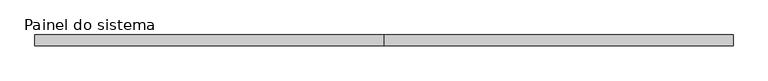
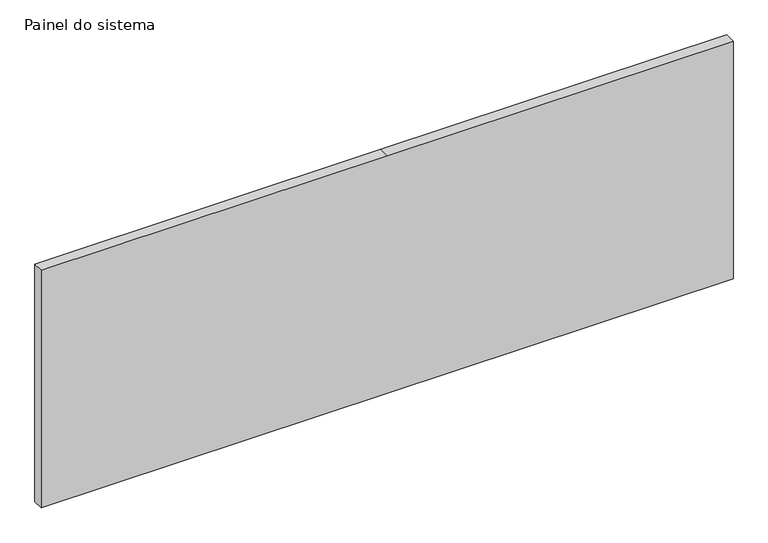
"""IFC4 building model written with IfcOpenShell, lengths in millimetres: plate geometry, Painel do sistema : Envidraçado."""

from ifc_helpers import new_model, si_unit, frame, origin, place, context, project, spatial, polyline, outline, extrude, source, transform, mapped, element, save


def painel_do_sistema_229e198e(model_context):
    return source(origin(), model_context, "Body", "SweptSolid", [
        extrude(outline(polyline([(0.0, -812.5499999), (0.0, 0.0), (0.0, 812.5499999), (590.0, 812.5499999), (590.0, 0.0), (590.0, -812.5499999), (0.0, -812.5499999)])), frame((0.0, -49.5, 0.0), z_axis=(0.0, 1.0, 0.0), x_axis=(0.0, 0.0, 1.0)), (0.0, 0.0, 1.0), 25.0),
    ])


if __name__ == "__main__":
    model = new_model("IFC4")
    model_context = context("Model", 3, world=origin())
    ifc_project = project(units=[si_unit("LENGTHUNIT", "METRE", prefix="MILLI")], contexts=[model_context])
    site = spatial("IfcSite", under=ifc_project)
    building = spatial("IfcBuilding", under=site)
    placement = place(None, origin())
    painel_do_sistema_shape = painel_do_sistema_229e198e(model_context)
    element("IfcPlate", 1, ObjectType="Painel do sistema : Envidraçado", at=placement, inside=building, context=model_context, shape_type="MappedRepresentation", body=[
        mapped(painel_do_sistema_shape, transform((0.0, 0.0, 0.0), x_axis=(1.0, 0.0, 0.0), y_axis=(0.0, 1.0, 0.0), z_axis=(0.0, 0.0, 1.0))),
    ])
    save(model, "model.ifc")

# Revit data of these elements
# Type "Painel do sistema : Envidraçado"
#   Construction Type Id = "GSP4R"
#   Analytic Construction = "Vidraça única Pilkington 1/8 pol"
#   Visual Light Transmittance = 0.9
#   Solar Heat Gain Coefficient = 0.86
#   Heat Transfer Coefficient (U) = 6.7069 W/(m²·K)
# Element 1 (IfcPlate, "Painel do sistema : Envidraçado")
#   Materials on its faces: ".VIDRO GENÉRICO"
# Materials
#   ".VIDRO GENÉRICO": class ".CC_VIDRO", colour RGB 0 128 192, transparency 0.9, Description = "Vidro comum", Cost = 0
